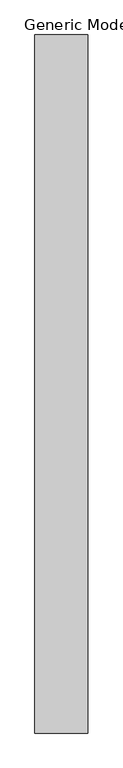
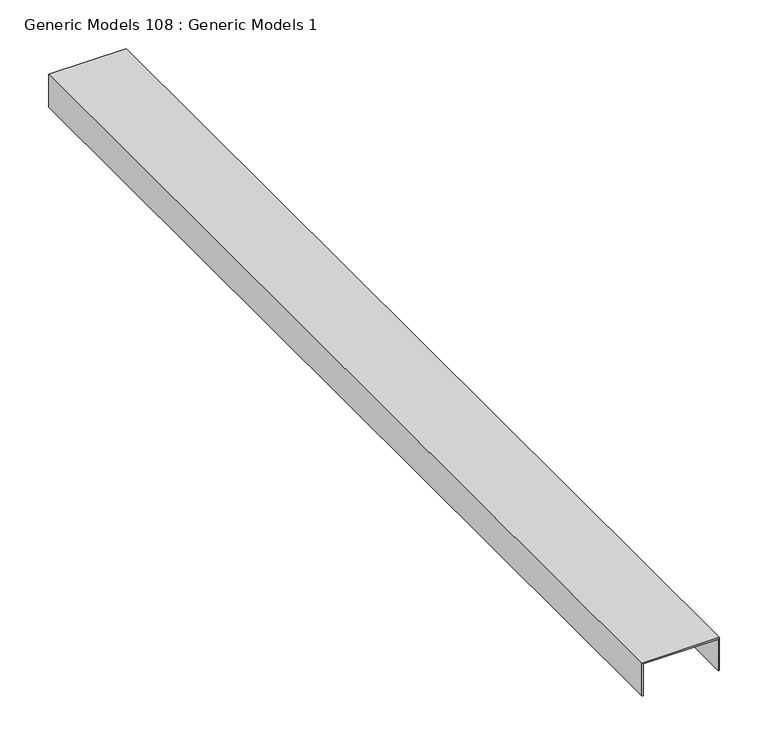
"""IFC4 building model written with IfcOpenShell, lengths in millimetres: proxy geometry, Generic Models 108 : Generic Models 1."""

from ifc_helpers import new_model, si_unit, frame, origin, place, context, project, spatial, polyline, outline, extrude, source, transform, mapped, element, save


def generic_models_108_generic_models_1_d2f1e0fb(model_context):
    return source(origin(), model_context, "Body", "SweptSolid", [
        extrude(outline(polyline([(2457.45, 49784.0), (2457.45, 49691.925), (2416.175, 49691.925), (2416.175, 49693.5125), (2455.8625, 49693.5125), (2455.8625, 49782.4125), (2416.175, 49782.4125), (2416.175, 49784.0), (2457.45, 49784.0)])), frame((0.0, 0.0, 0.0), z_axis=(0.0, 1.0, 0.0), x_axis=(0.0, 0.0, 1.0)), (0.0, 0.0, 1.0), 1219.2),
    ])


if __name__ == "__main__":
    model = new_model("IFC4")
    model_context = context("Model", 3, world=origin())
    ifc_project = project(units=[si_unit("LENGTHUNIT", "METRE", prefix="MILLI")], contexts=[model_context])
    site = spatial("IfcSite", under=ifc_project)
    building = spatial("IfcBuilding", under=site)
    placement = place(None, origin())
    generic_models_108_generic_models_1_shape = generic_models_108_generic_models_1_d2f1e0fb(model_context)
    element("IfcBuildingElementProxy", 1, Name="Generic Models 108 : Generic Models 1", ObjectType="Generic Models 108 : Generic Models 1", at=placement, inside=building, context=model_context, shape_type="MappedRepresentation", body=[
        mapped(generic_models_108_generic_models_1_shape, transform((0.0, 0.0, 0.0), x_axis=(1.0, 0.0, 0.0), y_axis=(0.0, 1.0, 0.0), z_axis=(0.0, 0.0, 1.0))),
    ])
    save(model, "model.ifc")

# Revit data of these elements
# Element 1 (IfcBuildingElementProxy, "Generic Models 108 : Generic Models 1")
#   Materials on its faces: "MATCH DEPTH OF EXISTING DEFLECTION TRACK"
# Materials
#   "MATCH DEPTH OF EXISTING DEFLECTION TRACK": class "Unassigned", colour RGB 210 209 208, transparency 0, Keynote = "M05121300.02", Cost = 0
